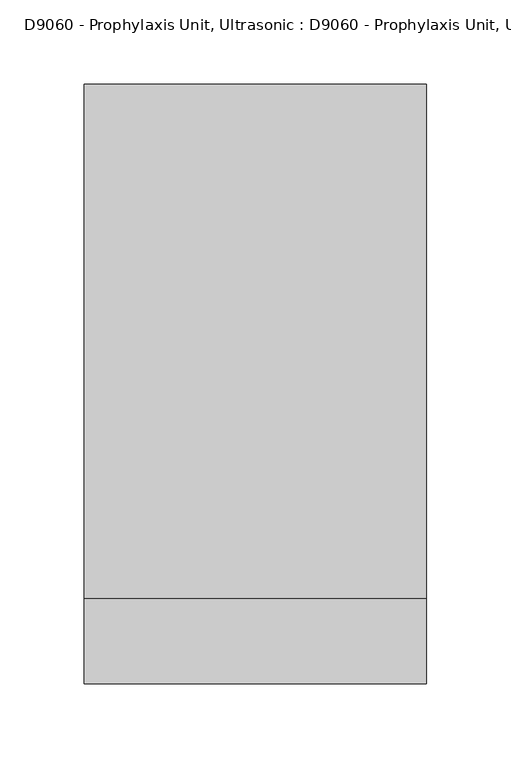
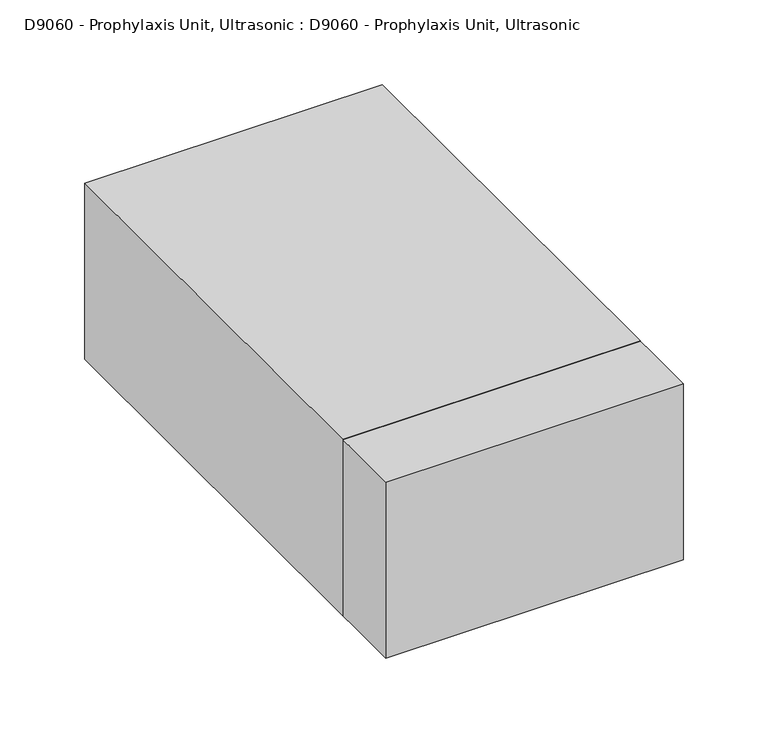
"""IFC4 building model written with IfcOpenShell, lengths in millimetres: proxy geometry, D9060 - Prophylaxis Unit, Ultrasonic : D9060 - Prophylaxis Unit, Ultrasonic."""

import ifcopenshell
import ifcopenshell.guid

model = None  # the IFC model being written
_history = None  # IfcOwnerHistory: only IFC2X3 demands one
_inside = {}  # id of a spatial element -> (the spatial element, [elements in it])
_under = {}  # id of a project, library or spatial element -> (it, [spatial elements below it])
_declared = {}  # id of a project -> (the project, [libraries it declares])
_typed = {}  # id of a type object -> (the type object, [elements of that type])
_made_of = {}  # id of a material, layer set ... -> (it, [elements and type objects made of it])


def new_model(schema):
    """Start an empty IFC model of exactly this schema.

    Asked for "IFC4X3", IfcOpenShell would pick the latest addendum, in which some entities
    have other attributes; the version numbers below select the first issue.
    IFC2X3 requires an IfcOwnerHistory on every rooted entity: one is made here for all.
    """
    global model, _history
    if schema == "IFC4X3":
        model = ifcopenshell.file(schema_version=(4, 3, 0, 0))
    else:
        model = ifcopenshell.file(schema=schema)
    _inside.clear()
    _under.clear()
    _declared.clear()
    _typed.clear()
    _made_of.clear()
    _history = None
    if model.schema == "IFC2X3":
        org = make("IfcOrganization", Name="unknown")
        user = make(
            "IfcPersonAndOrganization",
            ThePerson=make("IfcPerson", FamilyName="unknown"),
            TheOrganization=org,
        )
        app = make(
            "IfcApplication",
            ApplicationDeveloper=org,
            Version="unknown",
            ApplicationFullName="unknown",
            ApplicationIdentifier="unknown",
        )
        _history = make(
            "IfcOwnerHistory",
            OwningUser=user,
            OwningApplication=app,
            ChangeAction="ADDED",
            CreationDate=0,
        )
    return model


def make(cls, **values):
    """One entity of the class cls with the attributes given. An attribute that is None is left unset."""
    return model.create_entity(
        cls, **{name: value for name, value in values.items() if value is not None}
    )


def rooted(cls, **values):
    """An entity with a GlobalId (a new one), such as an element, a storey or a relation."""
    return make(cls, GlobalId=ifcopenshell.guid.new(), OwnerHistory=_history, **values)


def si_unit(unit_type, name, prefix=None):
    """IfcSIUnit, for example si_unit("LENGTHUNIT", "METRE", prefix="MILLI")."""
    return make("IfcSIUnit", UnitType=unit_type, Prefix=prefix, Name=name)


def assignment(units):
    """IfcUnitAssignment: the units of a project."""
    return None if units is None else make("IfcUnitAssignment", Units=units)


def point(xyz):
    """IfcCartesianPoint."""
    return None if xyz is None else make("IfcCartesianPoint", Coordinates=xyz)


def direction(xyz):
    """IfcDirection."""
    return None if xyz is None else make("IfcDirection", DirectionRatios=xyz)


def frame(location, z_axis=None, x_axis=None):
    """IfcAxis2Placement3D, a coordinate frame: its origin and axes. An axis left out is left unset."""
    return make(
        "IfcAxis2Placement3D",
        Location=point(location),
        Axis=direction(z_axis),
        RefDirection=direction(x_axis),
    )


def frame_2d(location, x_axis=None):
    """IfcAxis2Placement2D, a coordinate frame in the plane: its origin and x axis."""
    return make(
        "IfcAxis2Placement2D", Location=point(location), RefDirection=direction(x_axis)
    )


def origin():
    """The frame at (0, 0, 0) with its axes left unset."""
    return frame((0.0, 0.0, 0.0))


def origin_with_axes():
    """The frame at (0, 0, 0) with the z axis (0, 0, 1) and the x axis (1, 0, 0) written out."""
    return frame((0.0, 0.0, 0.0), z_axis=(0.0, 0.0, 1.0), x_axis=(1.0, 0.0, 0.0))


def place(relative_to, where):
    """IfcLocalPlacement: puts the frame where relative to a parent placement (None: the world)."""
    return make(
        "IfcLocalPlacement", PlacementRelTo=relative_to, RelativePlacement=where
    )


def context(
    kind, dimensions, precision=None, world=None, true_north=None, identifier=None
):
    """IfcGeometricRepresentationContext, for example the 3D "Model" context."""
    return make(
        "IfcGeometricRepresentationContext",
        ContextIdentifier=identifier,
        ContextType=kind,
        CoordinateSpaceDimension=dimensions,
        Precision=precision,
        WorldCoordinateSystem=world,
        TrueNorth=true_north,
    )


def project(units=None, contexts=None):
    """IfcProject with its units and contexts."""
    return rooted(
        "IfcProject",
        Name="project",
        RepresentationContexts=contexts,
        UnitsInContext=assignment(units),
    )


def spatial(cls, under=None, at=None, **own):
    """A site, building, storey or space (cls), placed at a placement, below another one or the project."""
    s = rooted(cls, ObjectPlacement=at, **own)
    if under is not None:
        _under.setdefault(under.id(), (under, []))[1].append(s)
    return s


def polyline(points):
    """IfcPolyline through the points."""
    return make("IfcPolyline", Points=[point(p) for p in points])


def circle_curve(where, radius):
    """IfcCircle in the frame where."""
    return make("IfcCircle", Position=where, Radius=radius)


def trimmed(basis, trim1, trim2, sense, master):
    """IfcTrimmedCurve: the piece of a basis curve between two trims."""
    return make(
        "IfcTrimmedCurve",
        BasisCurve=basis,
        Trim1=trim1,
        Trim2=trim2,
        SenseAgreement=sense,
        MasterRepresentation=master,
    )


def segment(curve, same_sense, transition):
    """IfcCompositeCurveSegment."""
    return make(
        "IfcCompositeCurveSegment",
        Transition=transition,
        SameSense=same_sense,
        ParentCurve=curve,
    )


def composite_curve(segments, self_intersect=None):
    """IfcCompositeCurve: segments joined end to end."""
    return make("IfcCompositeCurve", Segments=segments, SelfIntersect=self_intersect)


def outline(outer, holes=None, kind="AREA"):
    """IfcArbitraryClosedProfileDef: a profile drawn as a closed curve; with holes, ...WithVoids."""
    if holes is None:
        return make("IfcArbitraryClosedProfileDef", ProfileType=kind, OuterCurve=outer)
    return make(
        "IfcArbitraryProfileDefWithVoids",
        ProfileType=kind,
        OuterCurve=outer,
        InnerCurves=holes,
    )


def extrude(swept, where, along, depth):
    """IfcExtrudedAreaSolid: the profile swept, set in the frame where, extruded along a direction by depth."""
    return make(
        "IfcExtrudedAreaSolid",
        SweptArea=swept,
        Position=where,
        ExtrudedDirection=direction(along),
        Depth=depth,
    )


def shape(context_of_items, identifier, shape_type, items):
    """IfcShapeRepresentation: the items that make up one representation, for example the "Body"."""
    return make(
        "IfcShapeRepresentation",
        ContextOfItems=context_of_items,
        RepresentationIdentifier=identifier,
        RepresentationType=shape_type,
        Items=items,
    )


def source(mapping_origin, context_of_items, identifier, shape_type, items):
    """IfcRepresentationMap: a shape defined once, which mapped items show again and again."""
    return make(
        "IfcRepresentationMap",
        MappingOrigin=mapping_origin,
        MappedRepresentation=shape(context_of_items, identifier, shape_type, items),
    )


def transform(
    local_origin,
    x_axis=None,
    y_axis=None,
    z_axis=None,
    scale=None,
    scale2=None,
    scale3=None,
    uniform=True,
):
    """IfcCartesianTransformationOperator3D, or its non-uniform kind. x_axis, y_axis, z_axis: its Axis1, 2, 3."""
    if uniform:
        return make(
            "IfcCartesianTransformationOperator3D",
            Axis1=direction(x_axis),
            Axis2=direction(y_axis),
            LocalOrigin=point(local_origin),
            Scale=scale,
            Axis3=direction(z_axis),
        )
    return make(
        "IfcCartesianTransformationOperator3DnonUniform",
        Axis1=direction(x_axis),
        Axis2=direction(y_axis),
        LocalOrigin=point(local_origin),
        Scale=scale,
        Axis3=direction(z_axis),
        Scale2=scale2,
        Scale3=scale3,
    )


def mapped(mapping_source, mapping_target):
    """IfcMappedItem: shows the shape of a source again, moved by a transform."""
    return make(
        "IfcMappedItem", MappingSource=mapping_source, MappingTarget=mapping_target
    )


def made_of(thing, what):
    """Note that an element or type object is made of a material, layer set ...; save() writes the relation."""
    if what is not None:
        _made_of.setdefault(what.id(), (what, []))[1].append(thing)
    return thing


def element(
    cls,
    number,
    at=None,
    inside=None,
    cuts=None,
    type_object=None,
    material=None,
    context=None,
    identifier="Body",
    shape_type=None,
    held_by="IfcProductDefinitionShape",
    body=None,
    shapes=None,
    **own,
):
    """One element of the class cls, such as IfcWall. Its Tag is "e" and its number.

    at: its placement. inside: the storey or other place that contains it. cuts: it is an
    opening in that element (IfcRelVoidsElement). A single representation is given by context,
    identifier, shape_type and body (its items); several are given by shapes. held_by: the class
    of the entity that holds the representations. save() writes the other relations.
    """
    e = rooted(cls, Tag="e%d" % number, ObjectPlacement=at, **own)
    if body is not None:
        shapes = [shape(context, identifier, shape_type, body)]
    if shapes is not None:
        e.Representation = make(held_by, Representations=shapes)
    if inside is not None:
        _inside.setdefault(inside.id(), (inside, []))[1].append(e)
    if cuts is not None:
        rooted(
            "IfcRelVoidsElement", RelatingBuildingElement=cuts, RelatedOpeningElement=e
        )
    if type_object is not None:
        _typed.setdefault(type_object.id(), (type_object, []))[1].append(e)
    return made_of(e, material)


def aggregate(whole, parts):
    """IfcRelAggregates: a whole, such as a stair, and the parts it consists of."""
    return rooted("IfcRelAggregates", RelatingObject=whole, RelatedObjects=parts)


def save(model, path):
    """Write the relations noted so far, then the file.

    IfcRelAggregates (storeys below a building ...), IfcRelContainedInSpatialStructure (elements
    in a storey), IfcRelDefinesByType, IfcRelAssociatesMaterial and IfcRelDeclares: one each for
    every whole, place, type object, material and project.
    """
    for whole, parts in _under.values():
        aggregate(whole, parts)
    for where, things in _inside.values():
        rooted(
            "IfcRelContainedInSpatialStructure",
            RelatedElements=things,
            RelatingStructure=where,
        )
    for kind, things in _typed.values():
        rooted("IfcRelDefinesByType", RelatedObjects=things, RelatingType=kind)
    for what, things in _made_of.values():
        rooted("IfcRelAssociatesMaterial", RelatedObjects=things, RelatingMaterial=what)
    for by, libraries in _declared.values():
        rooted("IfcRelDeclares", RelatingContext=by, RelatedDefinitions=libraries)
    model.write(path)


def plane_surface(at):
    """IfcPlane: the flat surface through the origin of the frame at, square to its z axis."""
    return make("IfcPlane", Position=at)


def revolved_surface(curve, axis_point, axis_direction):
    """IfcSurfaceOfRevolution: the curve turned about the line through axis_point along axis_direction."""
    return make(
        "IfcSurfaceOfRevolution",
        SweptCurve=make("IfcArbitraryOpenProfileDef", ProfileType="CURVE", Curve=curve),
        AxisPosition=make("IfcAxis1Placement", Location=point(axis_point), Axis=direction(axis_direction)),
    )


def advanced_brep(points, edges, surfaces, faces):
    """IfcAdvancedBrep: a solid bounded by faces that lie on surfaces and meet in shared edges.

    An edge is (start, end): straight between two places in points (the first is 0);
    or (start, end, curve); or (start, end, curve, False) where it runs against its curve.
    A face is (place in surfaces, loops), or (place, loops, False) where it looks against
    its surface's normal. A loop lists edges by number (the first is 1), with a minus sign
    where the edge is run from its end to its start. The first loop is the outer one.
    """
    corners = [point(p) for p in points]
    vertices = [make("IfcVertexPoint", VertexGeometry=c) for c in corners]
    made = []
    for start, end, *more in edges:
        made.append(
            make(
                "IfcEdgeCurve",
                EdgeStart=vertices[start],
                EdgeEnd=vertices[end],
                EdgeGeometry=more[0] if more else make("IfcPolyline", Points=[corners[start], corners[end]]),
                SameSense=more[1] if len(more) > 1 else True,
            )
        )
    hull = []
    for where, loops, *sense in faces:
        bounds = []
        for j, loop in enumerate(loops):
            ring = [make("IfcOrientedEdge", EdgeElement=made[abs(k) - 1], Orientation=k > 0) for k in loop]
            bounds.append(
                make(
                    "IfcFaceOuterBound" if j == 0 else "IfcFaceBound",
                    Bound=make("IfcEdgeLoop", EdgeList=ring),
                    Orientation=True,
                )
            )
        hull.append(make("IfcAdvancedFace", Bounds=bounds, FaceSurface=surfaces[where], SameSense=sense[0] if sense else True))
    return make("IfcAdvancedBrep", Outer=make("IfcClosedShell", CfsFaces=hull))


def d9060_prophylaxis_unit_ultrasonic_d9060_prophylaxis_unit_4aaabe70(model_context):
    return source(origin(), model_context, "Body", "SolidModel", [
        advanced_brep(
        [(101.6, 177.8, 127.0), (-101.6, 177.8, 127.0), (-101.6, -127.0, 127.0), (101.6, -127.0, 127.0), (101.6, 177.8, 0.0), (101.6, -127.0, 0.0), (-101.6, -127.0, 0.0), (-101.6, 177.8, 0.0), (-33.3504232, -127.0, 26.6792148), (-46.0504232, -127.0, 26.6792148), (46.0504232, -127.0, 26.6792148), (33.3504232, -127.0, 26.6792148), (-46.0504232, -113.1251573, 26.6792148), (-33.3504232, -113.1251573, 26.6792148), (33.3504232, -113.1251573, 26.6792148), (46.0504232, -113.1251573, 26.6792148)],
        [
            (0, 1),
            (1, 2),
            (2, 3),
            (3, 0),
            (4, 5),
            (5, 6),
            (6, 7),
            (7, 4),
            (0, 4),
            (7, 1),
            (6, 2),
            (5, 3),
            (8, 9, circle_curve(frame((-39.7004232, -127.0, 26.6792148), z_axis=(0.0, 1.0, 0.0), x_axis=(1.0, 0.0, 0.0)), 6.35)),
            (9, 8, circle_curve(frame((-39.7004232, -127.0, 26.6792148), z_axis=(0.0, 1.0, 0.0), x_axis=(1.0, 0.0, 0.0)), 6.35)),
            (10, 11, circle_curve(frame((39.7004232, -127.0, 26.6792148), z_axis=(0.0, 1.0, 0.0), x_axis=(1.0, 0.0, 0.0)), 6.35)),
            (11, 10, circle_curve(frame((39.7004232, -127.0, 26.6792148), z_axis=(0.0, 1.0, 0.0), x_axis=(1.0, 0.0, 0.0)), 6.35)),
            (12, 13, circle_curve(frame((-39.7004232, -113.1251573, 26.6792148), z_axis=(0.0, -1.0, 0.0), x_axis=(1.0, 0.0, 0.0)), 6.35)),
            (13, 12, circle_curve(frame((-39.7004232, -113.1251573, 26.6792148), z_axis=(0.0, -1.0, 0.0), x_axis=(1.0, 0.0, 0.0)), 6.35)),
            (14, 15, circle_curve(frame((39.7004232, -113.1251573, 26.6792148), z_axis=(0.0, -1.0, 0.0), x_axis=(1.0, 0.0, 0.0)), 6.35)),
            (15, 14, circle_curve(frame((39.7004232, -113.1251573, 26.6792148), z_axis=(0.0, -1.0, 0.0), x_axis=(1.0, 0.0, 0.0)), 6.35)),
            (12, 9),
            (8, 13),
            (14, 11),
            (10, 15),
        ],
        [
            plane_surface(frame((-101.6, 177.8, 127.0), z_axis=(0.0, 0.0, 1.0), x_axis=(-1.0, 0.0, 0.0))),
            plane_surface(frame((-101.6, 177.8, 0.0), z_axis=(0.0, 0.0, -1.0), x_axis=(1.0, 0.0, 0.0))),
            plane_surface(frame((101.6, 177.8, 127.0), z_axis=(0.0, 1.0, 0.0), x_axis=(0.0, 0.0, -1.0))),
            plane_surface(frame((-101.6, 177.8, 127.0), z_axis=(-1.0, 0.0, 0.0), x_axis=(0.0, 0.0, -1.0))),
            plane_surface(frame((-101.6, -127.0, 127.0), z_axis=(0.0, -1.0, 0.0), x_axis=(0.0, 0.0, -1.0))),
            plane_surface(frame((101.6, -127.0, 127.0), z_axis=(1.0, 0.0, 0.0), x_axis=(0.0, 0.0, -1.0))),
            plane_surface(frame((-33.3504232, -113.1251573, 26.6792148), z_axis=(0.0, -1.0, 0.0), x_axis=(0.0, 0.0, -1.0))),
            revolved_surface(polyline([(-33.3504232, -127.0, 26.6792148), (-33.3504232, -113.1251573, 26.6792148)]), (-39.7004232, -113.1251573, 26.6792148), (0.0, -1.0, 0.0)),
            revolved_surface(polyline([(46.050423200000004, -126.99999999999999, 26.6792148), (46.050423200000004, -113.1251573, 26.6792148)]), (39.7004232, 13.8748427, 26.6792148), (0.0, -1.0, 0.0)),
        ],
        [
            (0, [[1, 2, 3, 4]]),
            (1, [[5, 6, 7, 8]]),
            (2, [[-1, 9, -8, 10]]),
            (3, [[-2, -10, -7, 11]]),
            (4, [[-3, -11, -6, 12], [13, 14], [15, 16]]),
            (5, [[-4, -12, -5, -9]]),
            (6, [[17, 18]]),
            (6, [[19, 20]]),
            (7, [[-17, 21, -13, 22]]),
            (7, [[-18, -22, -14, -21]]),
            (8, [[-19, 23, -15, 24]]),
            (8, [[-20, -24, -16, -23]]),
        ],
    ),
        extrude(outline(composite_curve([segment(trimmed(circle_curve(frame_2d((60.9232765, -73.6139431)), 12.7), [point((60.9232765, -86.3139431))], [point((60.9232765, -60.9139431))], False, "CARTESIAN"), True, "CONTINUOUS"), segment(trimmed(circle_curve(frame_2d((60.9232765, -73.6139431)), 12.7), [point((60.9232765, -60.9139431))], [point((60.9232765, -86.3139431))], False, "CARTESIAN"), True, "CONTINUOUS")], self_intersect=False)), frame((0.0, -152.4, 0.0), z_axis=(0.0, 1.0, 0.0), x_axis=(0.0, 0.0, 1.0)), (0.0, 0.0, 1.0), 25.4),
        extrude(outline(composite_curve([segment(trimmed(circle_curve(frame_2d((60.9232765, 73.6139431)), 12.7), [point((60.9232765, 60.9139431))], [point((60.9232765, 86.3139431))], False, "CARTESIAN"), True, "CONTINUOUS"), segment(trimmed(circle_curve(frame_2d((60.9232765, 73.6139431)), 12.7), [point((60.9232765, 86.3139431))], [point((60.9232765, 60.9139431))], False, "CARTESIAN"), True, "CONTINUOUS")], self_intersect=False)), frame((0.0, -152.4, 0.0), z_axis=(0.0, 1.0, 0.0), x_axis=(0.0, 0.0, 1.0)), (0.0, 0.0, 1.0), 25.4),
        extrude(outline(composite_curve([segment(trimmed(circle_curve(frame_2d((60.9232765, 0.0)), 12.7), [point((60.9232765, -12.7))], [point((60.9232765, 12.7))], False, "CARTESIAN"), True, "CONTINUOUS"), segment(trimmed(circle_curve(frame_2d((60.9232765, 0.0)), 12.7), [point((60.9232765, 12.7))], [point((60.9232765, -12.7))], False, "CARTESIAN"), True, "CONTINUOUS")], self_intersect=False)), frame((0.0, -152.4, 0.0), z_axis=(0.0, 1.0, 0.0), x_axis=(0.0, 0.0, 1.0)), (0.0, 0.0, 1.0), 25.4),
        extrude(outline(polyline([(-101.6, 177.8), (101.6, 177.8), (101.6, -177.8), (-101.6, -177.8), (-101.6, 0.0), (-101.6, 177.8)])), origin_with_axes(), (0.0, 0.0, 1.0), 127.0),
    ])


if __name__ == "__main__":
    model = new_model("IFC4")
    model_context = context("Model", 3, world=origin())
    ifc_project = project(units=[si_unit("LENGTHUNIT", "METRE", prefix="MILLI")], contexts=[model_context])
    site = spatial("IfcSite", under=ifc_project)
    building = spatial("IfcBuilding", under=site)
    placement = place(None, origin())
    d9060_prophylaxis_unit_ultrasonic_d9060_prophylaxis_unit_shape = d9060_prophylaxis_unit_ultrasonic_d9060_prophylaxis_unit_4aaabe70(model_context)
    element("IfcBuildingElementProxy", 1, Name="D9060 - Prophylaxis Unit, Ultrasonic : D9060 - Prophylaxis Unit, Ultrasonic", ObjectType="D9060 - Prophylaxis Unit, Ultrasonic : D9060 - Prophylaxis Unit, Ultrasonic", at=placement, inside=building, context=model_context, shape_type="MappedRepresentation", body=[
        mapped(d9060_prophylaxis_unit_ultrasonic_d9060_prophylaxis_unit_shape, transform((0.0, 0.0, 0.0), x_axis=(1.0, 0.0, 0.0), y_axis=(0.0, 1.0, 0.0), z_axis=(0.0, 0.0, 1.0))),
    ])
    save(model, "model.ifc")

# Revit data of these elements
# Project information
#   Room Abbreviation = "DNTG3"
#   Room Description = "Dental Treatment Room, Two Chair (DNTG3)"
#   Sheets - Total = "5"
#   Project Issue Date = "Issue Date"
#   Project Status = "Project Status"
#   Client Name = "Owner"
#   Project Address = "Enter address here"
#   Project Name = "Project Name"
#   Project Number = "Project Number"
#   Publication Date = "30-Jan-15"
# Type "D9060 - Prophylaxis Unit, Ultrasonic : D9060 - Prophylaxis Unit, Ultrasonic"
#   Watts2 = "0"
#   Watts1 = "240"
#   Unit_Issue = "EA"
#   UTIL_6_Misc = "-"
#   UTIL_5_NonMedGas = "-"
#   UTIL_4_MiscGas = "-"
#   UTIL_3_MedGas = "D"
#   UTIL_2_Elec = "A"
#   UTIL_1_WaterDrain = "J"
#   Nomenclature = "Prophylaxis Unit, Ultrasonic"
#   NSN = "6520010456407"
#   Location [instance default] = ""
#   JSN = "D9060"
#   Fund_Source_VA = "-"
#   Fund_Source_Navy = "-"
#   Fund_Source_Army = "-"
#   Fund_Source_AF = "-"
#   ELEC_Volts2 = "0"
#   ELEC_Volts1 = "120"
#   ELEC_Phase2 = "0"
#   ELEC_Phase1 = "1"
#   ELEC_HertzSwitch = "-1"
#   ELEC_HertzDependent = "0"
#   ELEC_Hertz = "60"
#   ELEC_Amps2 = "0"
#   ELEC_Amps1 = "2"
#   DetailDescription = "Dental ultrasonic prophylaxis unit. Used in dental clinics for the removal of calculus. Unit requires water and air supplies."
#   CAT_VA = "C"
#   CAT_Navy = "C"
#   CAT_IHS = "-"
#   CAT_Army = "C"
#   CAT_AF = "C"
#   BTUperhour = "0"
#   Weight_IP = 13
#   DIM_Width_IP = 0' - 8"
#   DIM_Height_IP = 0' - 5"
#   DIM_Depth_IP = 1' - 2"
# Element 1 (IfcBuildingElementProxy, "D9060 - Prophylaxis Unit, Ultrasonic : D9060 - Prophylaxis Unit, Ultrasonic")
#   Materials on its faces: "EquipSpace"
# Materials
#   "EquipSpace": class "Unassigned", colour RGB 221 217 195, transparency 0.5
